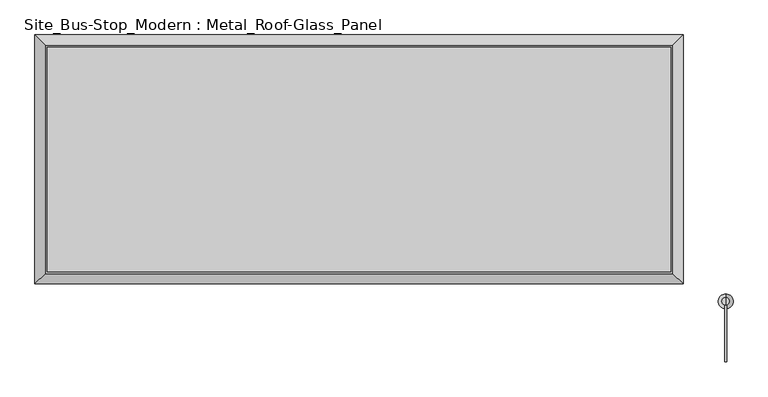
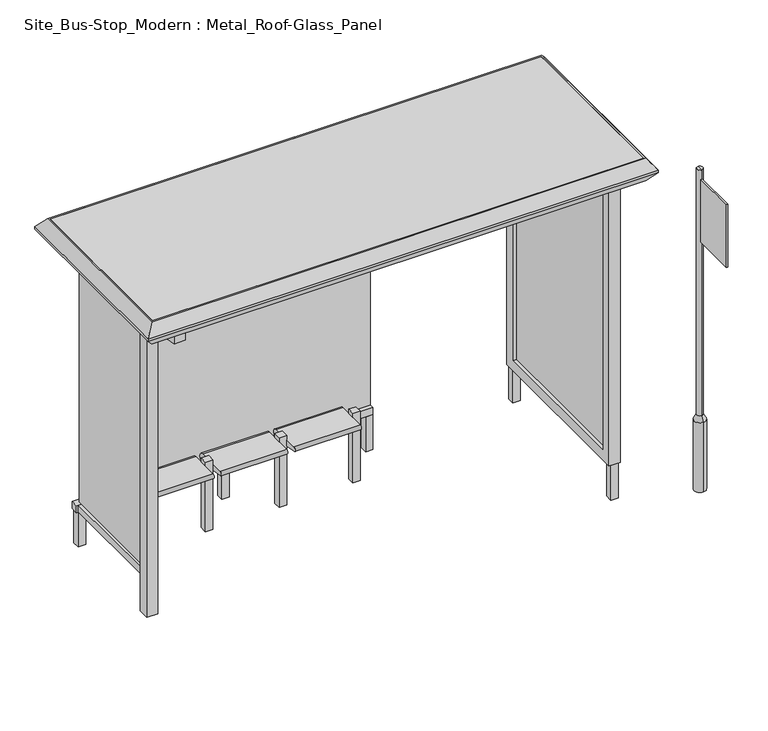
"""IFC4 building model written with IfcOpenShell, lengths in millimetres: geographic element geometry, Site_Bus-Stop_Modern : Metal_Roof-Glass_Panel."""

import ifcopenshell
import ifcopenshell.guid

model = None  # the IFC model being written
_history = None  # IfcOwnerHistory: only IFC2X3 demands one
_inside = {}  # id of a spatial element -> (the spatial element, [elements in it])
_under = {}  # id of a project, library or spatial element -> (it, [spatial elements below it])
_declared = {}  # id of a project -> (the project, [libraries it declares])
_typed = {}  # id of a type object -> (the type object, [elements of that type])
_made_of = {}  # id of a material, layer set ... -> (it, [elements and type objects made of it])


def new_model(schema):
    """Start an empty IFC model of exactly this schema.

    Asked for "IFC4X3", IfcOpenShell would pick the latest addendum, in which some entities
    have other attributes; the version numbers below select the first issue.
    IFC2X3 requires an IfcOwnerHistory on every rooted entity: one is made here for all.
    """
    global model, _history
    if schema == "IFC4X3":
        model = ifcopenshell.file(schema_version=(4, 3, 0, 0))
    else:
        model = ifcopenshell.file(schema=schema)
    _inside.clear()
    _under.clear()
    _declared.clear()
    _typed.clear()
    _made_of.clear()
    _history = None
    if model.schema == "IFC2X3":
        org = make("IfcOrganization", Name="unknown")
        user = make(
            "IfcPersonAndOrganization",
            ThePerson=make("IfcPerson", FamilyName="unknown"),
            TheOrganization=org,
        )
        app = make(
            "IfcApplication",
            ApplicationDeveloper=org,
            Version="unknown",
            ApplicationFullName="unknown",
            ApplicationIdentifier="unknown",
        )
        _history = make(
            "IfcOwnerHistory",
            OwningUser=user,
            OwningApplication=app,
            ChangeAction="ADDED",
            CreationDate=0,
        )
    return model


def make(cls, **values):
    """One entity of the class cls with the attributes given. An attribute that is None is left unset."""
    return model.create_entity(
        cls, **{name: value for name, value in values.items() if value is not None}
    )


def rooted(cls, **values):
    """An entity with a GlobalId (a new one), such as an element, a storey or a relation."""
    return make(cls, GlobalId=ifcopenshell.guid.new(), OwnerHistory=_history, **values)


def si_unit(unit_type, name, prefix=None):
    """IfcSIUnit, for example si_unit("LENGTHUNIT", "METRE", prefix="MILLI")."""
    return make("IfcSIUnit", UnitType=unit_type, Prefix=prefix, Name=name)


def assignment(units):
    """IfcUnitAssignment: the units of a project."""
    return None if units is None else make("IfcUnitAssignment", Units=units)


def point(xyz):
    """IfcCartesianPoint."""
    return None if xyz is None else make("IfcCartesianPoint", Coordinates=xyz)


def direction(xyz):
    """IfcDirection."""
    return None if xyz is None else make("IfcDirection", DirectionRatios=xyz)


def frame(location, z_axis=None, x_axis=None):
    """IfcAxis2Placement3D, a coordinate frame: its origin and axes. An axis left out is left unset."""
    return make(
        "IfcAxis2Placement3D",
        Location=point(location),
        Axis=direction(z_axis),
        RefDirection=direction(x_axis),
    )


def frame_2d(location, x_axis=None):
    """IfcAxis2Placement2D, a coordinate frame in the plane: its origin and x axis."""
    return make(
        "IfcAxis2Placement2D", Location=point(location), RefDirection=direction(x_axis)
    )


def origin():
    """The frame at (0, 0, 0) with its axes left unset."""
    return frame((0.0, 0.0, 0.0))


def origin_with_axes():
    """The frame at (0, 0, 0) with the z axis (0, 0, 1) and the x axis (1, 0, 0) written out."""
    return frame((0.0, 0.0, 0.0), z_axis=(0.0, 0.0, 1.0), x_axis=(1.0, 0.0, 0.0))


def place(relative_to, where):
    """IfcLocalPlacement: puts the frame where relative to a parent placement (None: the world)."""
    return make(
        "IfcLocalPlacement", PlacementRelTo=relative_to, RelativePlacement=where
    )


def context(
    kind, dimensions, precision=None, world=None, true_north=None, identifier=None
):
    """IfcGeometricRepresentationContext, for example the 3D "Model" context."""
    return make(
        "IfcGeometricRepresentationContext",
        ContextIdentifier=identifier,
        ContextType=kind,
        CoordinateSpaceDimension=dimensions,
        Precision=precision,
        WorldCoordinateSystem=world,
        TrueNorth=true_north,
    )


def project(units=None, contexts=None):
    """IfcProject with its units and contexts."""
    return rooted(
        "IfcProject",
        Name="project",
        RepresentationContexts=contexts,
        UnitsInContext=assignment(units),
    )


def spatial(cls, under=None, at=None, **own):
    """A site, building, storey or space (cls), placed at a placement, below another one or the project."""
    s = rooted(cls, ObjectPlacement=at, **own)
    if under is not None:
        _under.setdefault(under.id(), (under, []))[1].append(s)
    return s


def polyline(points):
    """IfcPolyline through the points."""
    return make("IfcPolyline", Points=[point(p) for p in points])


def circle_curve(where, radius):
    """IfcCircle in the frame where."""
    return make("IfcCircle", Position=where, Radius=radius)


def trimmed(basis, trim1, trim2, sense, master):
    """IfcTrimmedCurve: the piece of a basis curve between two trims."""
    return make(
        "IfcTrimmedCurve",
        BasisCurve=basis,
        Trim1=trim1,
        Trim2=trim2,
        SenseAgreement=sense,
        MasterRepresentation=master,
    )


def segment(curve, same_sense, transition):
    """IfcCompositeCurveSegment."""
    return make(
        "IfcCompositeCurveSegment",
        Transition=transition,
        SameSense=same_sense,
        ParentCurve=curve,
    )


def composite_curve(segments, self_intersect=None):
    """IfcCompositeCurve: segments joined end to end."""
    return make("IfcCompositeCurve", Segments=segments, SelfIntersect=self_intersect)


def outline(outer, holes=None, kind="AREA"):
    """IfcArbitraryClosedProfileDef: a profile drawn as a closed curve; with holes, ...WithVoids."""
    if holes is None:
        return make("IfcArbitraryClosedProfileDef", ProfileType=kind, OuterCurve=outer)
    return make(
        "IfcArbitraryProfileDefWithVoids",
        ProfileType=kind,
        OuterCurve=outer,
        InnerCurves=holes,
    )


def extrude(swept, where, along, depth):
    """IfcExtrudedAreaSolid: the profile swept, set in the frame where, extruded along a direction by depth."""
    return make(
        "IfcExtrudedAreaSolid",
        SweptArea=swept,
        Position=where,
        ExtrudedDirection=direction(along),
        Depth=depth,
    )


def faces_of(points, faces, orient=None, outer=None):
    """IfcFace entities. A face is a list of loops; a loop is a list of indices into points, from 0.

    orient and outer hold one flag for each loop. By default every Orientation is true, the
    first loop of a face is its IfcFaceOuterBound and the others are IfcFaceBound.
    """
    made = []
    for i, loops in enumerate(faces):
        bounds = []
        for j, loop in enumerate(loops):
            is_outer = j == 0 if outer is None else outer[i][j]
            bounds.append(
                make(
                    "IfcFaceOuterBound" if is_outer else "IfcFaceBound",
                    Bound=make("IfcPolyLoop", Polygon=[points[k] for k in loop]),
                    Orientation=True if orient is None else orient[i][j],
                )
            )
        made.append(make("IfcFace", Bounds=bounds))
    return made


def faceted_brep(points, faces, orient=None, outer=None, voids=None):
    """IfcFacetedBrep: a solid bounded by flat faces; with voids (closed shells), ...WithVoids."""
    shared = [point(p) for p in points]
    hull = make("IfcClosedShell", CfsFaces=faces_of(shared, faces, orient, outer))
    if voids is None:
        return make("IfcFacetedBrep", Outer=hull)
    return make(
        "IfcFacetedBrepWithVoids",
        Outer=hull,
        Voids=[
            make(cls, CfsFaces=faces_of(shared, fs, o, b)) for cls, fs, o, b in voids
        ],
    )


def shape(context_of_items, identifier, shape_type, items):
    """IfcShapeRepresentation: the items that make up one representation, for example the "Body"."""
    return make(
        "IfcShapeRepresentation",
        ContextOfItems=context_of_items,
        RepresentationIdentifier=identifier,
        RepresentationType=shape_type,
        Items=items,
    )


def source(mapping_origin, context_of_items, identifier, shape_type, items):
    """IfcRepresentationMap: a shape defined once, which mapped items show again and again."""
    return make(
        "IfcRepresentationMap",
        MappingOrigin=mapping_origin,
        MappedRepresentation=shape(context_of_items, identifier, shape_type, items),
    )


def transform(
    local_origin,
    x_axis=None,
    y_axis=None,
    z_axis=None,
    scale=None,
    scale2=None,
    scale3=None,
    uniform=True,
):
    """IfcCartesianTransformationOperator3D, or its non-uniform kind. x_axis, y_axis, z_axis: its Axis1, 2, 3."""
    if uniform:
        return make(
            "IfcCartesianTransformationOperator3D",
            Axis1=direction(x_axis),
            Axis2=direction(y_axis),
            LocalOrigin=point(local_origin),
            Scale=scale,
            Axis3=direction(z_axis),
        )
    return make(
        "IfcCartesianTransformationOperator3DnonUniform",
        Axis1=direction(x_axis),
        Axis2=direction(y_axis),
        LocalOrigin=point(local_origin),
        Scale=scale,
        Axis3=direction(z_axis),
        Scale2=scale2,
        Scale3=scale3,
    )


def mapped(mapping_source, mapping_target):
    """IfcMappedItem: shows the shape of a source again, moved by a transform."""
    return make(
        "IfcMappedItem", MappingSource=mapping_source, MappingTarget=mapping_target
    )


def made_of(thing, what):
    """Note that an element or type object is made of a material, layer set ...; save() writes the relation."""
    if what is not None:
        _made_of.setdefault(what.id(), (what, []))[1].append(thing)
    return thing


def element(
    cls,
    number,
    at=None,
    inside=None,
    cuts=None,
    type_object=None,
    material=None,
    context=None,
    identifier="Body",
    shape_type=None,
    held_by="IfcProductDefinitionShape",
    body=None,
    shapes=None,
    **own,
):
    """One element of the class cls, such as IfcWall. Its Tag is "e" and its number.

    at: its placement. inside: the storey or other place that contains it. cuts: it is an
    opening in that element (IfcRelVoidsElement). A single representation is given by context,
    identifier, shape_type and body (its items); several are given by shapes. held_by: the class
    of the entity that holds the representations. save() writes the other relations.
    """
    e = rooted(cls, Tag="e%d" % number, ObjectPlacement=at, **own)
    if body is not None:
        shapes = [shape(context, identifier, shape_type, body)]
    if shapes is not None:
        e.Representation = make(held_by, Representations=shapes)
    if inside is not None:
        _inside.setdefault(inside.id(), (inside, []))[1].append(e)
    if cuts is not None:
        rooted(
            "IfcRelVoidsElement", RelatingBuildingElement=cuts, RelatedOpeningElement=e
        )
    if type_object is not None:
        _typed.setdefault(type_object.id(), (type_object, []))[1].append(e)
    return made_of(e, material)


def aggregate(whole, parts):
    """IfcRelAggregates: a whole, such as a stair, and the parts it consists of."""
    return rooted("IfcRelAggregates", RelatingObject=whole, RelatedObjects=parts)


def save(model, path):
    """Write the relations noted so far, then the file.

    IfcRelAggregates (storeys below a building ...), IfcRelContainedInSpatialStructure (elements
    in a storey), IfcRelDefinesByType, IfcRelAssociatesMaterial and IfcRelDeclares: one each for
    every whole, place, type object, material and project.
    """
    for whole, parts in _under.values():
        aggregate(whole, parts)
    for where, things in _inside.values():
        rooted(
            "IfcRelContainedInSpatialStructure",
            RelatedElements=things,
            RelatingStructure=where,
        )
    for kind, things in _typed.values():
        rooted("IfcRelDefinesByType", RelatedObjects=things, RelatingType=kind)
    for what, things in _made_of.values():
        rooted("IfcRelAssociatesMaterial", RelatedObjects=things, RelatingMaterial=what)
    for by, libraries in _declared.values():
        rooted("IfcRelDeclares", RelatingContext=by, RelatedDefinitions=libraries)
    model.write(path)


def plane_surface(at):
    """IfcPlane: the flat surface through the origin of the frame at, square to its z axis."""
    return make("IfcPlane", Position=at)


def cylinder_surface(at, radius):
    """IfcCylindricalSurface: all points at the distance radius from the z axis of the frame at."""
    return make("IfcCylindricalSurface", Position=at, Radius=radius)


def revolved_surface(curve, axis_point, axis_direction):
    """IfcSurfaceOfRevolution: the curve turned about the line through axis_point along axis_direction."""
    return make(
        "IfcSurfaceOfRevolution",
        SweptCurve=make("IfcArbitraryOpenProfileDef", ProfileType="CURVE", Curve=curve),
        AxisPosition=make("IfcAxis1Placement", Location=point(axis_point), Axis=direction(axis_direction)),
    )


def advanced_brep(points, edges, surfaces, faces):
    """IfcAdvancedBrep: a solid bounded by faces that lie on surfaces and meet in shared edges.

    An edge is (start, end): straight between two places in points (the first is 0);
    or (start, end, curve); or (start, end, curve, False) where it runs against its curve.
    A face is (place in surfaces, loops), or (place, loops, False) where it looks against
    its surface's normal. A loop lists edges by number (the first is 1), with a minus sign
    where the edge is run from its end to its start. The first loop is the outer one.
    """
    corners = [point(p) for p in points]
    vertices = [make("IfcVertexPoint", VertexGeometry=c) for c in corners]
    made = []
    for start, end, *more in edges:
        made.append(
            make(
                "IfcEdgeCurve",
                EdgeStart=vertices[start],
                EdgeEnd=vertices[end],
                EdgeGeometry=more[0] if more else make("IfcPolyline", Points=[corners[start], corners[end]]),
                SameSense=more[1] if len(more) > 1 else True,
            )
        )
    hull = []
    for where, loops, *sense in faces:
        bounds = []
        for j, loop in enumerate(loops):
            ring = [make("IfcOrientedEdge", EdgeElement=made[abs(k) - 1], Orientation=k > 0) for k in loop]
            bounds.append(
                make(
                    "IfcFaceOuterBound" if j == 0 else "IfcFaceBound",
                    Bound=make("IfcEdgeLoop", EdgeList=ring),
                    Orientation=True,
                )
            )
        hull.append(make("IfcAdvancedFace", Bounds=bounds, FaceSurface=surfaces[where], SameSense=sense[0] if sense else True))
    return make("IfcAdvancedBrep", Outer=make("IfcClosedShell", CfsFaces=hull))


def site_bus_stop_modern_metal_roof_glass_panel_3fdf870d(model_context):
    return source(origin(), model_context, "Body", "SolidModel", [
        extrude(outline(polyline([(1957.5, -1680.3732439), (1957.5, -1380.3732439), (1967.5, -1380.3732439), (1967.5, -1680.3732439), (1957.5, -1680.3732439)])), frame((0.0, 0.0, 1784.6), z_axis=(0.0, 0.0, 1.0), x_axis=(1.0, 0.0, 0.0)), (0.0, 0.0, 1.0), 450.0),
        advanced_brep(
        [(1962.5, -1398.2604073, 500.0), (1962.5, -1318.2604073, 500.0), (1962.5, -1318.2604073, 0.0), (1962.5, -1398.2604073, 0.0), (1962.5, -1378.2604073, 534.6), (1962.5, -1338.2604073, 534.6), (1962.5, -1378.2604073, 2300.0), (1962.5, -1338.2604073, 2300.0), (1962.5, -1358.2604073, 2300.0), (1962.5, -1358.2604073, 0.0)],
        [
            (0, 1, circle_curve(frame((1962.5, -1358.2604073, 500.0), z_axis=(0.0, 0.0, -1.0), x_axis=(0.0, 1.0, 0.0)), 40.0)),
            (1, 2),
            (2, 3, circle_curve(frame((1962.5, -1358.2604073, 0.0), z_axis=(0.0, 0.0, 1.0), x_axis=(0.0, 1.0, 0.0)), 40.0)),
            (3, 0),
            (1, 0, circle_curve(frame((1962.5, -1358.2604073, 500.0), z_axis=(0.0, 0.0, -1.0), x_axis=(0.0, 1.0, 0.0)), 40.0)),
            (3, 2, circle_curve(frame((1962.5, -1358.2604073, 0.0), z_axis=(0.0, 0.0, 1.0), x_axis=(0.0, 1.0, 0.0)), 40.0)),
            (4, 5, circle_curve(frame((1962.5, -1358.2604073, 534.6), z_axis=(0.0, 0.0, -1.0), x_axis=(0.0, 1.0, 0.0)), 20.0)),
            (5, 1),
            (0, 4),
            (5, 4, circle_curve(frame((1962.5, -1358.2604073, 534.6), z_axis=(0.0, 0.0, -1.0), x_axis=(0.0, 1.0, 0.0)), 20.0)),
            (6, 7, circle_curve(frame((1962.5, -1358.2604073, 2300.0), z_axis=(0.0, 0.0, -1.0), x_axis=(0.0, 1.0, 0.0)), 20.0)),
            (7, 5),
            (4, 6),
            (7, 6, circle_curve(frame((1962.5, -1358.2604073, 2300.0), z_axis=(0.0, 0.0, -1.0), x_axis=(0.0, 1.0, 0.0)), 20.0)),
            (8, 7),
            (6, 8),
            (2, 9),
            (9, 3),
        ],
        [
            cylinder_surface(frame((1962.5, -1358.2604073, -120.0), z_axis=(0.0, 0.0, 1.0), x_axis=(0.0, 1.0, 0.0)), 40.0),
            revolved_surface(polyline([(1962.5, -1318.2604073, 500.0), (1962.5, -1338.2604073, 534.6)]), (1962.5, -1358.2604073, -120.0), (0.0, 0.0, 1.0)),
            cylinder_surface(frame((1962.5, -1358.2604073, -120.0), z_axis=(0.0, 0.0, 1.0), x_axis=(0.0, 1.0, 0.0)), 20.0),
            plane_surface(frame((1962.5, -1358.2604073, 2300.0), z_axis=(0.0, 0.0, 1.0), x_axis=(0.0, 1.0, 0.0))),
            plane_surface(frame((1962.5, -1358.2604073, 0.0), z_axis=(0.0, 0.0, -1.0), x_axis=(0.0, 1.0, 0.0))),
        ],
        [
            (0, [[1, 2, 3, 4]]),
            (0, [[5, -4, 6, -2]]),
            (1, [[7, 8, -1, 9]]),
            (1, [[10, -9, -5, -8]]),
            (2, [[11, 12, -7, 13]]),
            (2, [[14, -13, -10, -12]]),
            (3, [[15, -11, 16]]),
            (3, [[-16, -14, -15]]),
            (4, [[-3, 17, 18]]),
            (4, [[-6, -18, -17]]),
        ],
    ),
        faceted_brep([(1735.0, 65.0, 2310.0), (1680.0, 10.0, 2380.0), (1680.0, -1210.0, 2380.0), (1735.0, -1265.0, 2310.0), (1735.0, 65.0, 2290.0), (1735.0, -1265.0, 2290.0), (1680.0, 10.0, 2220.0), (1680.0, -1210.0, 2220.0), (1670.0, 0.0, 2380.0), (1670.0, 0.0, 2220.0), (1670.0, -1200.0, 2220.0), (1670.0, -1200.0, 2380.0), (-1672.5, -1210.0, 2380.0), (-1727.5, -1265.0, 2310.0), (-1727.5, -1265.0, 2290.0), (-1672.5, -1210.0, 2220.0), (-1662.5, -1200.0, 2220.0), (-1662.5, -1200.0, 2380.0), (-1672.5, 10.0, 2380.0), (-1727.5, 65.0, 2310.0), (-1727.5, 65.0, 2290.0), (-1672.5, 10.0, 2220.0), (-1662.5, 0.0, 2220.0), (-1662.5, 0.0, 2380.0)], [[[0, 1, 2, 3]], [[4, 0, 3, 5]], [[6, 4, 5, 7]], [[8, 9, 10, 11]], [[3, 2, 12, 13]], [[5, 3, 13, 14]], [[7, 5, 14, 15]], [[11, 10, 16, 17]], [[13, 12, 18, 19]], [[14, 13, 19, 20]], [[15, 14, 20, 21]], [[17, 16, 22, 23]], [[19, 18, 1, 0]], [[20, 19, 0, 4]], [[21, 20, 4, 6]], [[7, 15, 21, 6], [9, 22, 16, 10]], [[23, 22, 9, 8]], [[1, 18, 12, 2], [11, 17, 23, 8]]]),
        extrude(outline(polyline([(-1662.5, -1200.0), (-1662.5, 0.0), (1670.0, 0.0), (1670.0, -1200.0), (-1662.5, -1200.0)])), frame((0.0, 0.0, 2220.0), z_axis=(0.0, 0.0, 1.0), x_axis=(1.0, 0.0, 0.0)), (0.0, 0.0, 1.0), 160.0),
        extrude(outline(polyline([(1490.0, -50.0), (1490.0, -1150.0), (1480.0, -1150.0), (1480.0, -50.0), (1490.0, -50.0)])), frame((0.0, 0.0, 300.0), z_axis=(0.0, 0.0, 1.0), x_axis=(1.0, 0.0, 0.0)), (0.0, 0.0, 1.0), 1870.0),
        extrude(outline(polyline([(1460.0, -1150.0), (1460.0, -50.0), (1470.0, -50.0), (1470.0, -1150.0), (1460.0, -1150.0)])), frame((0.0, 0.0, 300.0), z_axis=(0.0, 0.0, 1.0), x_axis=(1.0, 0.0, 0.0)), (0.0, 0.0, 1.0), 1870.0),
        faceted_brep([(1512.5, 0.0, 250.0), (1437.5, 0.0, 250.0), (1437.5, 0.0, 2220.0), (1512.5, 0.0, 2220.0), (1487.5, -75.0, 325.0), (1512.5, -75.0, 325.0), (1512.5, -75.0, 2145.0), (1487.5, -75.0, 2145.0), (1462.5, -50.0, 300.0), (1487.5, -50.0, 300.0), (1487.5, -50.0, 2170.0), (1462.5, -50.0, 2170.0), (1437.5, -75.0, 325.0), (1462.5, -75.0, 325.0), (1462.5, -75.0, 2145.0), (1437.5, -75.0, 2145.0), (1437.5, -1200.0, 2220.0), (1512.5, -1200.0, 2220.0), (1512.5, -1125.0, 2145.0), (1487.5, -1125.0, 2145.0), (1487.5, -1150.0, 2170.0), (1462.5, -1150.0, 2170.0), (1462.5, -1125.0, 2145.0), (1437.5, -1125.0, 2145.0), (1437.5, -1200.0, 250.0), (1512.5, -1200.0, 250.0), (1512.5, -1125.0, 325.0), (1487.5, -1125.0, 325.0), (1487.5, -1150.0, 300.0), (1462.5, -1150.0, 300.0), (1462.5, -1125.0, 325.0), (1437.5, -1125.0, 325.0)], [[[0, 1, 2, 3]], [[4, 5, 6, 7]], [[8, 9, 10, 11]], [[12, 13, 14, 15]], [[3, 2, 16, 17]], [[7, 6, 18, 19]], [[11, 10, 20, 21]], [[15, 14, 22, 23]], [[17, 16, 24, 25]], [[19, 18, 26, 27]], [[21, 20, 28, 29]], [[23, 22, 30, 31]], [[25, 24, 1, 0]], [[3, 17, 25, 0], [5, 26, 18, 6]], [[27, 26, 5, 4]], [[9, 28, 20, 10], [7, 19, 27, 4]], [[29, 28, 9, 8]], [[11, 21, 29, 8], [13, 30, 22, 14]], [[31, 30, 13, 12]], [[1, 24, 16, 2], [15, 23, 31, 12]]]),
        extrude(outline(polyline([(500.0, -20.0), (-1470.0, -20.0), (-1470.0, -10.0), (500.0, -10.0), (500.0, -20.0)])), frame((0.0, 0.0, 300.0), z_axis=(0.0, 0.0, 1.0), x_axis=(1.0, 0.0, 0.0)), (0.0, 0.0, 1.0), 1920.0),
        extrude(outline(polyline([(-800.0, 300.0), (-800.0, 2100.0), (-25.0, 2158.125), (-25.0, 300.0), (-800.0, 300.0)])), frame((-1480.0, 0.0, 0.0), z_axis=(1.0, 0.0, 0.0), x_axis=(0.0, 1.0, 0.0)), (0.0, 0.0, 1.0), 10.0),
        extrude(outline(composite_curve([segment(trimmed(circle_curve(frame_2d((-171.5367578, 436.9988667)), 33.0011333), [point((-171.5367578, 470.0))], [point((-171.5367578, 403.9977334))], False, "CARTESIAN"), True, "CONTINUOUS"), segment(polyline([(-171.5367578, 403.9977334), (-376.5367578, 440.1447644)]), True, "CONTINUOUS"), segment(trimmed(circle_curve(frame_2d((-376.5367578, 455.0723822)), 14.9276178), [point((-376.5367578, 440.1447644))], [point((-376.5367578, 470.0))], False, "CARTESIAN"), True, "CONTINUOUS"), segment(polyline([(-376.5367578, 470.0), (-171.5367578, 470.0)]), True, "CONTINUOUS")], self_intersect=False)), frame((-225.0, 0.0, 0.0), z_axis=(1.0, 0.0, 0.0), x_axis=(0.0, 1.0, 0.0)), (0.0, 0.0, 1.0), 450.0),
        extrude(outline(composite_curve([segment(trimmed(circle_curve(frame_2d((-171.5367578, 436.9988667)), 33.0011333), [point((-171.5367578, 470.0))], [point((-171.5367578, 403.9977334))], False, "CARTESIAN"), True, "CONTINUOUS"), segment(polyline([(-171.5367578, 403.9977334), (-376.5367578, 440.1447644)]), True, "CONTINUOUS"), segment(trimmed(circle_curve(frame_2d((-376.5367578, 455.0723822)), 14.9276178), [point((-376.5367578, 440.1447644))], [point((-376.5367578, 470.0))], False, "CARTESIAN"), True, "CONTINUOUS"), segment(polyline([(-376.5367578, 470.0), (-171.5367578, 470.0)]), True, "CONTINUOUS")], self_intersect=False)), frame((-725.0, 0.0, 0.0), z_axis=(1.0, 0.0, 0.0), x_axis=(0.0, 1.0, 0.0)), (0.0, 0.0, 1.0), 450.0),
        extrude(outline(composite_curve([segment(trimmed(circle_curve(frame_2d((-173.0011333, 436.9988667)), 33.0011333), [point((-173.0011333, 470.0))], [point((-173.0011333, 403.9977334))], False, "CARTESIAN"), True, "CONTINUOUS"), segment(polyline([(-173.0011333, 403.9977334), (-378.0011333, 440.1447644)]), True, "CONTINUOUS"), segment(trimmed(circle_curve(frame_2d((-378.0011333, 455.0723822)), 14.9276178), [point((-378.0011333, 440.1447644))], [point((-378.0011333, 470.0))], False, "CARTESIAN"), True, "CONTINUOUS"), segment(polyline([(-378.0011333, 470.0), (-173.0011333, 470.0)]), True, "CONTINUOUS")], self_intersect=False)), frame((-1225.0, 0.0, 0.0), z_axis=(1.0, 0.0, 0.0), x_axis=(0.0, 1.0, 0.0)), (0.0, 0.0, 1.0), 450.0),
        extrude(outline(polyline([(-1200.0, 2220.0), (0.0, 2220.0), (0.0, 2160.0), (-800.0, 2100.0), (-875.0, 2100.0), (-1200.0, 2160.0), (-1200.0, 2220.0)])), frame((-1512.5, 0.0, 0.0), z_axis=(1.0, 0.0, 0.0), x_axis=(0.0, 1.0, 0.0)), (0.0, 0.0, 1.0), 75.0),
        extrude(outline(polyline([(-1437.5, -800.0), (-1437.5, -875.0), (-1512.5, -875.0), (-1512.5, -800.0), (-1437.5, -800.0)])), origin_with_axes(), (0.0, 0.0, 1.0), 2100.0),
        extrude(outline(polyline([(-1500.0, -50.0), (-1450.0, -50.0), (-1450.0, -800.0), (-1500.0, -800.0), (-1500.0, -50.0)])), frame((0.0, 0.0, 250.0), z_axis=(0.0, 0.0, 1.0), x_axis=(1.0, 0.0, 0.0)), (0.0, 0.0, 1.0), 50.0),
        extrude(outline(polyline([(500.0, 0.0), (500.0, -50.0), (-1512.5, -50.0), (-1512.5, 0.0), (500.0, 0.0)])), frame((0.0, 0.0, 250.0), z_axis=(0.0, 0.0, 1.0), x_axis=(1.0, 0.0, 0.0)), (0.0, 0.0, 1.0), 50.0),
        extrude(outline(polyline([(275.0, -240.0), (275.0, -290.0), (225.0, -290.0), (225.0, -240.0), (275.0, -240.0)])), origin_with_axes(), (0.0, 0.0, 1.0), 500.0),
        extrude(outline(polyline([(-225.0, -240.0), (-225.0, -290.0), (-275.0, -290.0), (-275.0, -240.0), (-225.0, -240.0)])), origin_with_axes(), (0.0, 0.0, 1.0), 500.0),
        extrude(outline(polyline([(-725.0, -240.0), (-725.0, -290.0), (-775.0, -290.0), (-775.0, -240.0), (-725.0, -240.0)])), origin_with_axes(), (0.0, 0.0, 1.0), 500.0),
        extrude(outline(polyline([(-1225.0, -240.0), (-1225.0, -290.0), (-1275.0, -290.0), (-1275.0, -240.0), (-1225.0, -240.0)])), origin_with_axes(), (0.0, 0.0, 1.0), 500.0),
        extrude(outline(polyline([(1500.0, -1150.0), (1500.0, -1200.0), (1450.0, -1200.0), (1450.0, -1150.0), (1500.0, -1150.0)])), origin_with_axes(), (0.0, 0.0, 1.0), 250.0),
        extrude(outline(polyline([(1500.0, 0.0), (1500.0, -50.0), (1450.0, -50.0), (1450.0, 0.0), (1500.0, 0.0)])), origin_with_axes(), (0.0, 0.0, 1.0), 250.0),
        extrude(outline(polyline([(500.0, 0.0), (500.0, -50.0), (450.0, -50.0), (450.0, 0.0), (500.0, 0.0)])), origin_with_axes(), (0.0, 0.0, 1.0), 250.0),
        extrude(outline(polyline([(-475.0, 0.0), (-475.0, -50.0), (-525.0, -50.0), (-525.0, 0.0), (-475.0, 0.0)])), origin_with_axes(), (0.0, 0.0, 1.0), 250.0),
        extrude(outline(polyline([(-1450.0, 0.0), (-1450.0, -50.0), (-1500.0, -50.0), (-1500.0, 0.0), (-1450.0, 0.0)])), origin_with_axes(), (0.0, 0.0, 1.0), 250.0),
    ])


if __name__ == "__main__":
    model = new_model("IFC4")
    model_context = context("Model", 3, world=origin())
    ifc_project = project(units=[si_unit("LENGTHUNIT", "METRE", prefix="MILLI")], contexts=[model_context])
    site = spatial("IfcSite", under=ifc_project)
    building = spatial("IfcBuilding", under=site)
    placement = place(None, origin())
    site_bus_stop_modern_metal_roof_glass_panel_shape = site_bus_stop_modern_metal_roof_glass_panel_3fdf870d(model_context)
    element("IfcGeographicElement", 1, ObjectType="Site_Bus-Stop_Modern : Metal_Roof-Glass_Panel", at=placement, inside=building, context=model_context, shape_type="MappedRepresentation", body=[
        mapped(site_bus_stop_modern_metal_roof_glass_panel_shape, transform((0.0, 0.0, 0.0), x_axis=(1.0, 0.0, 0.0), y_axis=(0.0, 1.0, 0.0), z_axis=(0.0, 0.0, 1.0))),
    ])
    save(model, "model.ifc")

# Revit data of these elements
# Type "Site_Bus-Stop_Modern : Metal_Roof-Glass_Panel"
#   Material Structure = Metal - Aluminium Satin Hammered
#   Material Seat = Plastic - Red Light Textured
#   Material Roof = Metal - Aluminium Satin
#   Material Bus Stop Sign = Plastic - White Smooth
#   Material Bus Stop Post = Paint - Grey Medium
#   Material Glass = Glass - Blue Dark
# Element 1 (IfcGeographicElement, "Site_Bus-Stop_Modern : Metal_Roof-Glass_Panel")
#   Materials on its faces: "Metal - Aluminium Satin Hammered", "Glass - Blue Dark", "Metal - Aluminium Satin", "Plastic - Red Light Textured", "Paint - Grey Medium", "Plastic - White Smooth"
# Materials
#   "Metal - Aluminium Satin Hammered": class "Metal", colour RGB 247 247 247, transparency 0
#   "Plastic - Red Light Textured": class "Plastic", colour RGB 247 135 0, transparency 0
#   "Metal - Aluminium Satin": class "Metal", colour RGB 247 247 247, transparency 0
#   "Plastic - White Smooth": class "Plastic", colour RGB 249 249 249, transparency 0
#   "Paint - Grey Medium": class "Paint", colour RGB 162 162 162, transparency 0
#   "Glass - Blue Dark": class "Glass", colour RGB 57 95 150, transparency 0.7
